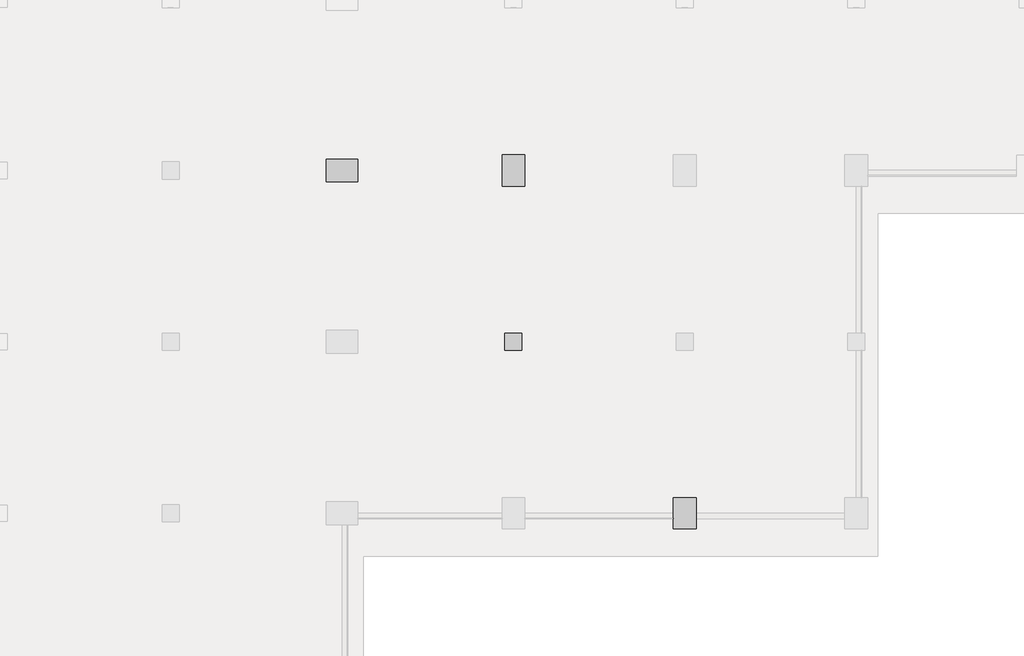
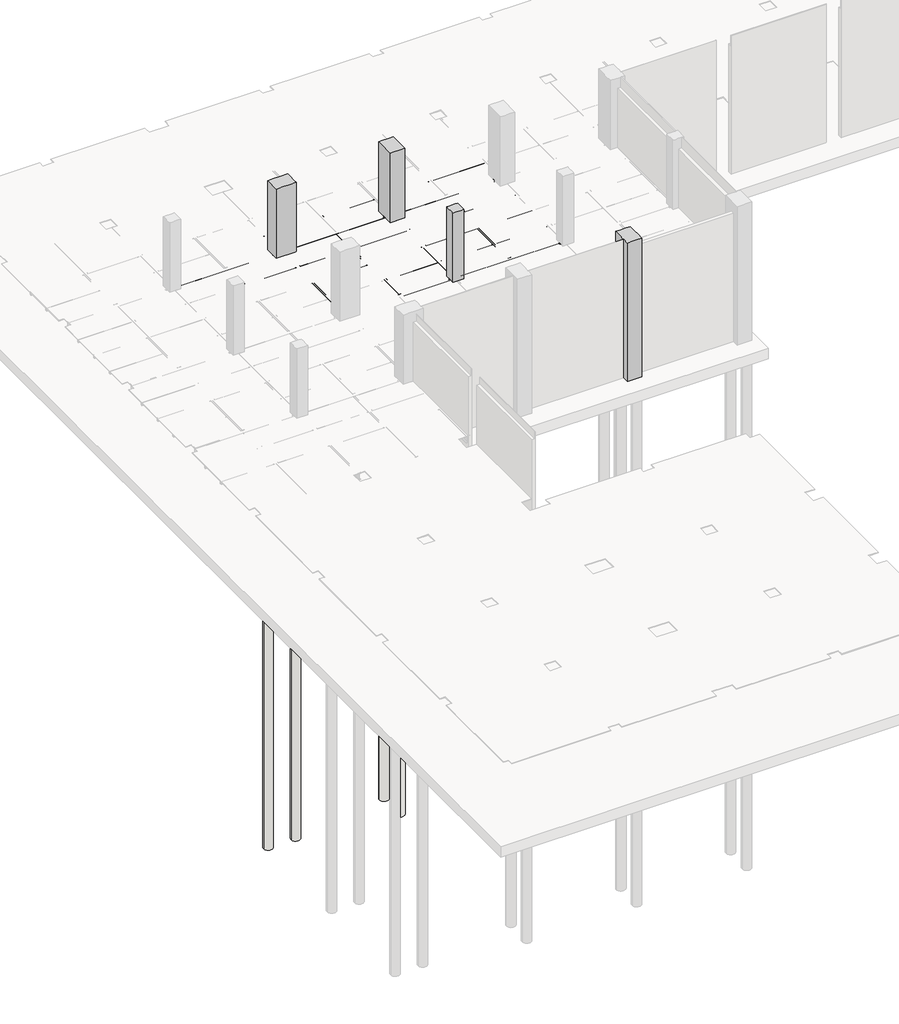
# Not in any storey, part 10 of 16: 28 beams, 6 slabs, 4 columns.
"""IFC4 building model written with IfcOpenShell, lengths in millimetres."""

from ifc_helpers import new_model, si_unit, point, frame, frame_2d, origin, place, context, project, spatial, polyline, circle_curve, trimmed, segment, composite_curve, outline, extrude, faceted_brep, element, save

model = new_model("IFC4")

# Units and contexts
model_context = context("Model", 3, world=origin())
ifc_project = project(units=[si_unit("LENGTHUNIT", "METRE", prefix="MILLI")], contexts=[model_context])

# Site, building
site = spatial("IfcSite", under=ifc_project)
building = spatial("IfcBuilding", under=site)

# Beams
placement = place(None, origin())
element("IfcBeam", 1, ObjectType="Steel Framing_H_KS : H_SB_AR_S02_H-400x200x8x13_BSG1", at=placement, inside=building, context=model_context, shape_type="SweptSolid", body=[
    extrude(outline(composite_curve([segment(polyline([(-17900.0, -4187.0381366), (-17900.0, -4200.0381366), (-18100.0, -4200.0381366), (-18100.0, -4187.0381366), (-18020.0, -4187.0381366)]), True, "CONTINUOUS"), segment(trimmed(circle_curve(frame_2d((-18020.0, -4171.0381366)), 16.0), [point((-18020.0, -4187.0381366))], [point((-18004.0, -4171.0381366))], True, "CARTESIAN"), True, "CONTINUOUS"), segment(polyline([(-18004.0, -4171.0381366), (-18004.0, -3829.0381366)]), True, "CONTINUOUS"), segment(trimmed(circle_curve(frame_2d((-18020.0, -3829.0381366)), 16.0), [point((-18004.0, -3829.0381366))], [point((-18020.0, -3813.0381366))], True, "CARTESIAN"), True, "CONTINUOUS"), segment(polyline([(-18020.0, -3813.0381366), (-18100.0, -3813.0381366), (-18100.0, -3800.0381366), (-17900.0, -3800.0381366), (-17900.0, -3813.0381366), (-17980.0, -3813.0381366)]), True, "CONTINUOUS"), segment(trimmed(circle_curve(frame_2d((-17980.0, -3829.0381366)), 16.0), [point((-17980.0, -3813.0381366))], [point((-17996.0, -3829.0381366))], True, "CARTESIAN"), True, "CONTINUOUS"), segment(polyline([(-17996.0, -3829.0381366), (-17996.0, -4171.0381366)]), True, "CONTINUOUS"), segment(trimmed(circle_curve(frame_2d((-17980.0, -4171.0381366)), 16.0), [point((-17996.0, -4171.0381366))], [point((-17980.0, -4187.0381366))], True, "CARTESIAN"), True, "CONTINUOUS"), segment(polyline([(-17980.0, -4187.0381366), (-17900.0, -4187.0381366)]), True, "CONTINUOUS")], self_intersect=False)), frame((30312.7, 0.0, 0.0), z_axis=(1.0, 0.0, 0.0), x_axis=(0.0, 1.0, 0.0)), (0.0, 0.0, 1.0), 5124.6),
])
element("IfcBeam", 2, ObjectType="Steel Framing_C_KS : H_SB_AR_S02_C-150x75x6.5x10_J1", at=placement, inside=building, context=model_context, shape_type="SweptSolid", body=[
    extrude(outline(composite_curve([segment(polyline([(-16477.2, -3800.0381366), (-16477.2, -3950.0381366), (-16552.2, -3950.0381366)]), True, "CONTINUOUS"), segment(trimmed(circle_curve(frame_2d((-16542.2, -3950.0381366)), 10.0), [point((-16552.2, -3950.0381366))], [point((-16542.2, -3940.0381366))], False, "CARTESIAN"), True, "CONTINUOUS"), segment(polyline([(-16542.2, -3940.0381366), (-16483.7, -3930.7726469), (-16483.7, -3819.3036264), (-16542.2, -3810.0381366)]), True, "CONTINUOUS"), segment(trimmed(circle_curve(frame_2d((-16542.2, -3800.0381366)), 10.0), [point((-16542.2, -3810.0381366))], [point((-16552.2, -3800.0381366))], False, "CARTESIAN"), True, "CONTINUOUS"), segment(polyline([(-16552.2, -3800.0381366), (-16477.2, -3800.0381366)]), True, "CONTINUOUS")], self_intersect=False)), frame((33112.7, 0.0, 0.0), z_axis=(1.0, 0.0, 0.0), x_axis=(0.0, 1.0, 0.0)), (0.0, 0.0, 1.0), 2774.6),
])
element("IfcBeam", 3, ObjectType="Steel Framing_H_KS : H_SB_AR_S02_H-400x200x8x13_BSG1", at=placement, inside=building, context=model_context, shape_type="SweptSolid", body=[
    extrude(outline(composite_curve([segment(polyline([(-17900.0, -4187.0381366), (-17900.0, -4200.0381366), (-18100.0, -4200.0381366), (-18100.0, -4187.0381366), (-18020.0, -4187.0381366)]), True, "CONTINUOUS"), segment(trimmed(circle_curve(frame_2d((-18020.0, -4171.0381366)), 16.0), [point((-18020.0, -4187.0381366))], [point((-18004.0, -4171.0381366))], True, "CARTESIAN"), True, "CONTINUOUS"), segment(polyline([(-18004.0, -4171.0381366), (-18004.0, -3829.0381366)]), True, "CONTINUOUS"), segment(trimmed(circle_curve(frame_2d((-18020.0, -3829.0381366)), 16.0), [point((-18004.0, -3829.0381366))], [point((-18020.0, -3813.0381366))], True, "CARTESIAN"), True, "CONTINUOUS"), segment(polyline([(-18020.0, -3813.0381366), (-18100.0, -3813.0381366), (-18100.0, -3800.0381366), (-17900.0, -3800.0381366), (-17900.0, -3813.0381366), (-17980.0, -3813.0381366)]), True, "CONTINUOUS"), segment(trimmed(circle_curve(frame_2d((-17980.0, -3829.0381366)), 16.0), [point((-17980.0, -3813.0381366))], [point((-17996.0, -3829.0381366))], True, "CARTESIAN"), True, "CONTINUOUS"), segment(polyline([(-17996.0, -3829.0381366), (-17996.0, -4171.0381366)]), True, "CONTINUOUS"), segment(trimmed(circle_curve(frame_2d((-17980.0, -4171.0381366)), 16.0), [point((-17996.0, -4171.0381366))], [point((-17980.0, -4187.0381366))], True, "CARTESIAN"), True, "CONTINUOUS"), segment(polyline([(-17980.0, -4187.0381366), (-17900.0, -4187.0381366)]), True, "CONTINUOUS")], self_intersect=False)), frame((36562.7, 0.0, 0.0), z_axis=(1.0, 0.0, 0.0), x_axis=(0.0, 1.0, 0.0)), (0.0, 0.0, 1.0), 5024.6),
])
element("IfcBeam", 4, ObjectType="Steel Framing_C_KS : H_SB_AR_S02_C-150x75x6.5x10_J1", at=placement, inside=building, context=model_context, shape_type="SweptSolid", body=[
    extrude(outline(composite_curve([segment(polyline([(-16477.2, -3800.0381366), (-16477.2, -3950.0381366), (-16552.2, -3950.0381366)]), True, "CONTINUOUS"), segment(trimmed(circle_curve(frame_2d((-16542.2, -3950.0381366)), 10.0), [point((-16552.2, -3950.0381366))], [point((-16542.2, -3940.0381366))], False, "CARTESIAN"), True, "CONTINUOUS"), segment(polyline([(-16542.2, -3940.0381366), (-16483.7, -3930.7726469), (-16483.7, -3819.3036264), (-16542.2, -3810.0381366)]), True, "CONTINUOUS"), segment(trimmed(circle_curve(frame_2d((-16542.2, -3800.0381366)), 10.0), [point((-16542.2, -3810.0381366))], [point((-16552.2, -3800.0381366))], False, "CARTESIAN"), True, "CONTINUOUS"), segment(polyline([(-16552.2, -3800.0381366), (-16477.2, -3800.0381366)]), True, "CONTINUOUS")], self_intersect=False)), frame((36112.7, 0.0, 0.0), z_axis=(1.0, 0.0, 0.0), x_axis=(0.0, 1.0, 0.0)), (0.0, 0.0, 1.0), 2774.6),
])
element("IfcBeam", 5, ObjectType="Steel Framing_C_KS : H_SB_AR_S02_C-150x75x6.5x10_J1", at=placement, inside=building, context=model_context, shape_type="SweptSolid", body=[
    extrude(outline(composite_curve([segment(polyline([(-16477.2, -3800.0381366), (-16477.2, -3950.0381366), (-16552.2, -3950.0381366)]), True, "CONTINUOUS"), segment(trimmed(circle_curve(frame_2d((-16542.2, -3950.0381366)), 10.0), [point((-16552.2, -3950.0381366))], [point((-16542.2, -3940.0381366))], False, "CARTESIAN"), True, "CONTINUOUS"), segment(polyline([(-16542.2, -3940.0381366), (-16483.7, -3930.7726469), (-16483.7, -3819.3036264), (-16542.2, -3810.0381366)]), True, "CONTINUOUS"), segment(trimmed(circle_curve(frame_2d((-16542.2, -3800.0381366)), 10.0), [point((-16542.2, -3810.0381366))], [point((-16552.2, -3800.0381366))], False, "CARTESIAN"), True, "CONTINUOUS"), segment(polyline([(-16552.2, -3800.0381366), (-16477.2, -3800.0381366)]), True, "CONTINUOUS")], self_intersect=False)), frame((39112.7, 0.0, 0.0), z_axis=(1.0, 0.0, 0.0), x_axis=(0.0, 1.0, 0.0)), (0.0, 0.0, 1.0), 2774.6),
])
element("IfcBeam", 6, ObjectType="Steel Framing_H_KS : H_SB_AR_S02_H-400x200x8x13_BSG1", at=placement, inside=building, context=model_context, shape_type="SweptSolid", body=[
    extrude(outline(composite_curve([segment(polyline([(-17900.0, -4187.0381366), (-17900.0, -4200.0381366), (-18100.0, -4200.0381366), (-18100.0, -4187.0381366), (-18020.0, -4187.0381366)]), True, "CONTINUOUS"), segment(trimmed(circle_curve(frame_2d((-18020.0, -4171.0381366)), 16.0), [point((-18020.0, -4187.0381366))], [point((-18004.0, -4171.0381366))], True, "CARTESIAN"), True, "CONTINUOUS"), segment(polyline([(-18004.0, -4171.0381366), (-18004.0, -3829.0381366)]), True, "CONTINUOUS"), segment(trimmed(circle_curve(frame_2d((-18020.0, -3829.0381366)), 16.0), [point((-18004.0, -3829.0381366))], [point((-18020.0, -3813.0381366))], True, "CARTESIAN"), True, "CONTINUOUS"), segment(polyline([(-18020.0, -3813.0381366), (-18100.0, -3813.0381366), (-18100.0, -3800.0381366), (-17900.0, -3800.0381366), (-17900.0, -3813.0381366), (-17980.0, -3813.0381366)]), True, "CONTINUOUS"), segment(trimmed(circle_curve(frame_2d((-17980.0, -3829.0381366)), 16.0), [point((-17980.0, -3813.0381366))], [point((-17996.0, -3829.0381366))], True, "CARTESIAN"), True, "CONTINUOUS"), segment(polyline([(-17996.0, -3829.0381366), (-17996.0, -4171.0381366)]), True, "CONTINUOUS"), segment(trimmed(circle_curve(frame_2d((-17980.0, -4171.0381366)), 16.0), [point((-17996.0, -4171.0381366))], [point((-17980.0, -4187.0381366))], True, "CARTESIAN"), True, "CONTINUOUS"), segment(polyline([(-17980.0, -4187.0381366), (-17900.0, -4187.0381366)]), True, "CONTINUOUS")], self_intersect=False)), frame((42412.7, 0.0, 0.0), z_axis=(1.0, 0.0, 0.0), x_axis=(0.0, 1.0, 0.0)), (0.0, 0.0, 1.0), 5174.6),
])
element("IfcBeam", 7, ObjectType="Steel Framing_C_KS : H_SB_AR_S02_C-150x75x6.5x10_J1", at=placement, inside=building, context=model_context, shape_type="SweptSolid", body=[
    extrude(outline(composite_curve([segment(polyline([(-16477.2, -3800.0381366), (-16477.2, -3950.0381366), (-16552.2, -3950.0381366)]), True, "CONTINUOUS"), segment(trimmed(circle_curve(frame_2d((-16542.2, -3950.0381366)), 10.0), [point((-16552.2, -3950.0381366))], [point((-16542.2, -3940.0381366))], False, "CARTESIAN"), True, "CONTINUOUS"), segment(polyline([(-16542.2, -3940.0381366), (-16483.7, -3930.7726469), (-16483.7, -3819.3036264), (-16542.2, -3810.0381366)]), True, "CONTINUOUS"), segment(trimmed(circle_curve(frame_2d((-16542.2, -3800.0381366)), 10.0), [point((-16542.2, -3810.0381366))], [point((-16552.2, -3800.0381366))], False, "CARTESIAN"), True, "CONTINUOUS"), segment(polyline([(-16552.2, -3800.0381366), (-16477.2, -3800.0381366)]), True, "CONTINUOUS")], self_intersect=False)), frame((42112.7, 0.0, 0.0), z_axis=(1.0, 0.0, 0.0), x_axis=(0.0, 1.0, 0.0)), (0.0, 0.0, 1.0), 2774.6),
])
element("IfcBeam", 8, ObjectType="Steel Framing_C_KS : H_SB_AR_S02_C-150x75x6.5x10_J1", at=placement, inside=building, context=model_context, shape_type="SweptSolid", body=[
    extrude(outline(composite_curve([segment(polyline([(-16477.2, -3800.0381366), (-16477.2, -3950.0381366), (-16552.2, -3950.0381366)]), True, "CONTINUOUS"), segment(trimmed(circle_curve(frame_2d((-16542.2, -3950.0381366)), 10.0), [point((-16552.2, -3950.0381366))], [point((-16542.2, -3940.0381366))], False, "CARTESIAN"), True, "CONTINUOUS"), segment(polyline([(-16542.2, -3940.0381366), (-16483.7, -3930.7726469), (-16483.7, -3819.3036264), (-16542.2, -3810.0381366)]), True, "CONTINUOUS"), segment(trimmed(circle_curve(frame_2d((-16542.2, -3800.0381366)), 10.0), [point((-16542.2, -3810.0381366))], [point((-16552.2, -3800.0381366))], False, "CARTESIAN"), True, "CONTINUOUS"), segment(polyline([(-16552.2, -3800.0381366), (-16477.2, -3800.0381366)]), True, "CONTINUOUS")], self_intersect=False)), frame((45112.7, 0.0, 0.0), z_axis=(1.0, 0.0, 0.0), x_axis=(0.0, 1.0, 0.0)), (0.0, 0.0, 1.0), 2774.6),
])
element("IfcBeam", 9, ObjectType="Steel Framing_H_KS : H_SB_AR_S02_H-400x200x8x13_BSG2", at=placement, inside=building, context=model_context, shape_type="SweptSolid", body=[
    extrude(outline(composite_curve([segment(polyline([(-4187.0381366, 35900.0), (-4200.0381366, 35900.0), (-4200.0381366, 36100.0), (-4187.0381366, 36100.0), (-4187.0381366, 36020.0)]), True, "CONTINUOUS"), segment(trimmed(circle_curve(frame_2d((-4171.0381366, 36020.0)), 16.0), [point((-4187.0381366, 36020.0))], [point((-4171.0381366, 36004.0))], True, "CARTESIAN"), True, "CONTINUOUS"), segment(polyline([(-4171.0381366, 36004.0), (-3829.0381366, 36004.0)]), True, "CONTINUOUS"), segment(trimmed(circle_curve(frame_2d((-3829.0381366, 36020.0)), 16.0), [point((-3829.0381366, 36004.0))], [point((-3813.0381366, 36020.0))], True, "CARTESIAN"), True, "CONTINUOUS"), segment(polyline([(-3813.0381366, 36020.0), (-3813.0381366, 36100.0), (-3800.0381366, 36100.0), (-3800.0381366, 35900.0), (-3813.0381366, 35900.0), (-3813.0381366, 35980.0)]), True, "CONTINUOUS"), segment(trimmed(circle_curve(frame_2d((-3829.0381366, 35980.0)), 16.0), [point((-3813.0381366, 35980.0))], [point((-3829.0381366, 35996.0))], True, "CARTESIAN"), True, "CONTINUOUS"), segment(polyline([(-3829.0381366, 35996.0), (-4171.0381366, 35996.0)]), True, "CONTINUOUS"), segment(trimmed(circle_curve(frame_2d((-4171.0381366, 35980.0)), 16.0), [point((-4171.0381366, 35996.0))], [point((-4187.0381366, 35980.0))], True, "CARTESIAN"), True, "CONTINUOUS"), segment(polyline([(-4187.0381366, 35980.0), (-4187.0381366, 35900.0)]), True, "CONTINUOUS")], self_intersect=False)), frame((0.0, -23587.3, 0.0), z_axis=(0.0, 1.0, 0.0), x_axis=(0.0, 0.0, 1.0)), (0.0, 0.0, 1.0), 5174.6),
])
element("IfcBeam", 10, ObjectType="Steel Framing_C_KS : H_SB_AR_S02_C-150x75x6.5x10_J1", at=placement, inside=building, context=model_context, shape_type="SweptSolid", body=[
    extrude(outline(composite_curve([segment(polyline([(-19477.2, -3800.0381366), (-19477.2, -3950.0381366), (-19552.2, -3950.0381366)]), True, "CONTINUOUS"), segment(trimmed(circle_curve(frame_2d((-19542.2, -3950.0381366)), 10.0), [point((-19552.2, -3950.0381366))], [point((-19542.2, -3940.0381366))], False, "CARTESIAN"), True, "CONTINUOUS"), segment(polyline([(-19542.2, -3940.0381366), (-19483.7, -3930.7726469), (-19483.7, -3819.3036264), (-19542.2, -3810.0381366)]), True, "CONTINUOUS"), segment(trimmed(circle_curve(frame_2d((-19542.2, -3800.0381366)), 10.0), [point((-19542.2, -3810.0381366))], [point((-19552.2, -3800.0381366))], False, "CARTESIAN"), True, "CONTINUOUS"), segment(polyline([(-19552.2, -3800.0381366), (-19477.2, -3800.0381366)]), True, "CONTINUOUS")], self_intersect=False)), frame((33112.7, 0.0, 0.0), z_axis=(1.0, 0.0, 0.0), x_axis=(0.0, 1.0, 0.0)), (0.0, 0.0, 1.0), 2774.6),
])
element("IfcBeam", 11, ObjectType="Steel Framing_H_KS : H_SB_AR_S02_H-400x200x8x13_BSG1", at=placement, inside=building, context=model_context, shape_type="SweptSolid", body=[
    extrude(outline(composite_curve([segment(polyline([(-23900.0, -4187.0381366), (-23900.0, -4200.0381366), (-24100.0, -4200.0381366), (-24100.0, -4187.0381366), (-24020.0, -4187.0381366)]), True, "CONTINUOUS"), segment(trimmed(circle_curve(frame_2d((-24020.0, -4171.0381366)), 16.0), [point((-24020.0, -4187.0381366))], [point((-24004.0, -4171.0381366))], True, "CARTESIAN"), True, "CONTINUOUS"), segment(polyline([(-24004.0, -4171.0381366), (-24004.0, -3829.0381366)]), True, "CONTINUOUS"), segment(trimmed(circle_curve(frame_2d((-24020.0, -3829.0381366)), 16.0), [point((-24004.0, -3829.0381366))], [point((-24020.0, -3813.0381366))], True, "CARTESIAN"), True, "CONTINUOUS"), segment(polyline([(-24020.0, -3813.0381366), (-24100.0, -3813.0381366), (-24100.0, -3800.0381366), (-23900.0, -3800.0381366), (-23900.0, -3813.0381366), (-23980.0, -3813.0381366)]), True, "CONTINUOUS"), segment(trimmed(circle_curve(frame_2d((-23980.0, -3829.0381366)), 16.0), [point((-23980.0, -3813.0381366))], [point((-23996.0, -3829.0381366))], True, "CARTESIAN"), True, "CONTINUOUS"), segment(polyline([(-23996.0, -3829.0381366), (-23996.0, -4171.0381366)]), True, "CONTINUOUS"), segment(trimmed(circle_curve(frame_2d((-23980.0, -4171.0381366)), 16.0), [point((-23996.0, -4171.0381366))], [point((-23980.0, -4187.0381366))], True, "CARTESIAN"), True, "CONTINUOUS"), segment(polyline([(-23980.0, -4187.0381366), (-23900.0, -4187.0381366)]), True, "CONTINUOUS")], self_intersect=False)), frame((36562.7, 0.0, 0.0), z_axis=(1.0, 0.0, 0.0), x_axis=(0.0, 1.0, 0.0)), (0.0, 0.0, 1.0), 5124.6),
])
element("IfcBeam", 12, ObjectType="Steel Framing_H_KS : H_SB_AR_S02_H-400x200x8x13_BSG2", at=placement, inside=building, context=model_context, shape_type="SweptSolid", body=[
    extrude(outline(composite_curve([segment(polyline([(-4187.0381366, 41900.0), (-4200.0381366, 41900.0), (-4200.0381366, 42100.0), (-4187.0381366, 42100.0), (-4187.0381366, 42020.0)]), True, "CONTINUOUS"), segment(trimmed(circle_curve(frame_2d((-4171.0381366, 42020.0)), 16.0), [point((-4187.0381366, 42020.0))], [point((-4171.0381366, 42004.0))], True, "CARTESIAN"), True, "CONTINUOUS"), segment(polyline([(-4171.0381366, 42004.0), (-3829.0381366, 42004.0)]), True, "CONTINUOUS"), segment(trimmed(circle_curve(frame_2d((-3829.0381366, 42020.0)), 16.0), [point((-3829.0381366, 42004.0))], [point((-3813.0381366, 42020.0))], True, "CARTESIAN"), True, "CONTINUOUS"), segment(polyline([(-3813.0381366, 42020.0), (-3813.0381366, 42100.0), (-3800.0381366, 42100.0), (-3800.0381366, 41900.0), (-3813.0381366, 41900.0), (-3813.0381366, 41980.0)]), True, "CONTINUOUS"), segment(trimmed(circle_curve(frame_2d((-3829.0381366, 41980.0)), 16.0), [point((-3813.0381366, 41980.0))], [point((-3829.0381366, 41996.0))], True, "CARTESIAN"), True, "CONTINUOUS"), segment(polyline([(-3829.0381366, 41996.0), (-4171.0381366, 41996.0)]), True, "CONTINUOUS"), segment(trimmed(circle_curve(frame_2d((-4171.0381366, 41980.0)), 16.0), [point((-4171.0381366, 41996.0))], [point((-4187.0381366, 41980.0))], True, "CARTESIAN"), True, "CONTINUOUS"), segment(polyline([(-4187.0381366, 41980.0), (-4187.0381366, 41900.0)]), True, "CONTINUOUS")], self_intersect=False)), frame((0.0, -23687.3, 0.0), z_axis=(0.0, 1.0, 0.0), x_axis=(0.0, 0.0, 1.0)), (0.0, 0.0, 1.0), 5124.6),
])
element("IfcBeam", 13, ObjectType="Steel Framing_H_KS : H_SB_AR_S02_H-400x200x8x13_BSB1", at=placement, inside=building, context=model_context, shape_type="SweptSolid", body=[
    extrude(outline(composite_curve([segment(polyline([(-4187.0381366, 38900.0), (-4200.0381366, 38900.0), (-4200.0381366, 39100.0), (-4187.0381366, 39100.0), (-4187.0381366, 39020.0)]), True, "CONTINUOUS"), segment(trimmed(circle_curve(frame_2d((-4171.0381366, 39020.0)), 16.0), [point((-4187.0381366, 39020.0))], [point((-4171.0381366, 39004.0))], True, "CARTESIAN"), True, "CONTINUOUS"), segment(polyline([(-4171.0381366, 39004.0), (-3829.0381366, 39004.0)]), True, "CONTINUOUS"), segment(trimmed(circle_curve(frame_2d((-3829.0381366, 39020.0)), 16.0), [point((-3829.0381366, 39004.0))], [point((-3813.0381366, 39020.0))], True, "CARTESIAN"), True, "CONTINUOUS"), segment(polyline([(-3813.0381366, 39020.0), (-3813.0381366, 39100.0), (-3800.0381366, 39100.0), (-3800.0381366, 38900.0), (-3813.0381366, 38900.0), (-3813.0381366, 38980.0)]), True, "CONTINUOUS"), segment(trimmed(circle_curve(frame_2d((-3829.0381366, 38980.0)), 16.0), [point((-3813.0381366, 38980.0))], [point((-3829.0381366, 38996.0))], True, "CARTESIAN"), True, "CONTINUOUS"), segment(polyline([(-3829.0381366, 38996.0), (-4171.0381366, 38996.0)]), True, "CONTINUOUS"), segment(trimmed(circle_curve(frame_2d((-4171.0381366, 38980.0)), 16.0), [point((-4171.0381366, 38996.0))], [point((-4187.0381366, 38980.0))], True, "CARTESIAN"), True, "CONTINUOUS"), segment(polyline([(-4187.0381366, 38980.0), (-4187.0381366, 38900.0)]), True, "CONTINUOUS")], self_intersect=False)), frame((0.0, -23887.3, 0.0), z_axis=(0.0, 1.0, 0.0), x_axis=(0.0, 0.0, 1.0)), (0.0, 0.0, 1.0), 5774.6),
])
element("IfcBeam", 14, ObjectType="Steel Framing_C_KS : H_SB_AR_S02_C-150x75x6.5x10_J1", at=placement, inside=building, context=model_context, shape_type="SweptSolid", body=[
    extrude(outline(composite_curve([segment(polyline([(-20977.2, -3800.0381366), (-20977.2, -3950.0381366), (-21052.2, -3950.0381366)]), True, "CONTINUOUS"), segment(trimmed(circle_curve(frame_2d((-21042.2, -3950.0381366)), 10.0), [point((-21052.2, -3950.0381366))], [point((-21042.2, -3940.0381366))], False, "CARTESIAN"), True, "CONTINUOUS"), segment(polyline([(-21042.2, -3940.0381366), (-20983.7, -3930.7726469), (-20983.7, -3819.3036264), (-21042.2, -3810.0381366)]), True, "CONTINUOUS"), segment(trimmed(circle_curve(frame_2d((-21042.2, -3800.0381366)), 10.0), [point((-21042.2, -3810.0381366))], [point((-21052.2, -3800.0381366))], False, "CARTESIAN"), True, "CONTINUOUS"), segment(polyline([(-21052.2, -3800.0381366), (-20977.2, -3800.0381366)]), True, "CONTINUOUS")], self_intersect=False)), frame((36112.7, 0.0, 0.0), z_axis=(1.0, 0.0, 0.0), x_axis=(0.0, 1.0, 0.0)), (0.0, 0.0, 1.0), 2774.6),
])
element("IfcBeam", 15, ObjectType="Steel Framing_C_KS : H_SB_AR_S02_C-150x75x6.5x10_J1", at=placement, inside=building, context=model_context, shape_type="SweptSolid", body=[
    extrude(outline(composite_curve([segment(polyline([(-19477.2, -3800.0381366), (-19477.2, -3950.0381366), (-19552.2, -3950.0381366)]), True, "CONTINUOUS"), segment(trimmed(circle_curve(frame_2d((-19542.2, -3950.0381366)), 10.0), [point((-19552.2, -3950.0381366))], [point((-19542.2, -3940.0381366))], False, "CARTESIAN"), True, "CONTINUOUS"), segment(polyline([(-19542.2, -3940.0381366), (-19483.7, -3930.7726469), (-19483.7, -3819.3036264), (-19542.2, -3810.0381366)]), True, "CONTINUOUS"), segment(trimmed(circle_curve(frame_2d((-19542.2, -3800.0381366)), 10.0), [point((-19542.2, -3810.0381366))], [point((-19552.2, -3800.0381366))], False, "CARTESIAN"), True, "CONTINUOUS"), segment(polyline([(-19552.2, -3800.0381366), (-19477.2, -3800.0381366)]), True, "CONTINUOUS")], self_intersect=False)), frame((36112.7, 0.0, 0.0), z_axis=(1.0, 0.0, 0.0), x_axis=(0.0, 1.0, 0.0)), (0.0, 0.0, 1.0), 2774.6),
])
element("IfcBeam", 16, ObjectType="Steel Framing_C_KS : H_SB_AR_S02_C-150x75x6.5x10_J1", at=placement, inside=building, context=model_context, shape_type="SweptSolid", body=[
    extrude(outline(composite_curve([segment(polyline([(-20977.2, -3800.0381366), (-20977.2, -3950.0381366), (-21052.2, -3950.0381366)]), True, "CONTINUOUS"), segment(trimmed(circle_curve(frame_2d((-21042.2, -3950.0381366)), 10.0), [point((-21052.2, -3950.0381366))], [point((-21042.2, -3940.0381366))], False, "CARTESIAN"), True, "CONTINUOUS"), segment(polyline([(-21042.2, -3940.0381366), (-20983.7, -3930.7726469), (-20983.7, -3819.3036264), (-21042.2, -3810.0381366)]), True, "CONTINUOUS"), segment(trimmed(circle_curve(frame_2d((-21042.2, -3800.0381366)), 10.0), [point((-21042.2, -3810.0381366))], [point((-21052.2, -3800.0381366))], False, "CARTESIAN"), True, "CONTINUOUS"), segment(polyline([(-21052.2, -3800.0381366), (-20977.2, -3800.0381366)]), True, "CONTINUOUS")], self_intersect=False)), frame((39112.7, 0.0, 0.0), z_axis=(1.0, 0.0, 0.0), x_axis=(0.0, 1.0, 0.0)), (0.0, 0.0, 1.0), 2774.6),
])
element("IfcBeam", 17, ObjectType="Steel Framing_C_KS : H_SB_AR_S02_C-150x75x6.5x10_J1", at=placement, inside=building, context=model_context, shape_type="SweptSolid", body=[
    extrude(outline(composite_curve([segment(polyline([(-22477.2, -3800.0381366), (-22477.2, -3950.0381366), (-22552.2, -3950.0381366)]), True, "CONTINUOUS"), segment(trimmed(circle_curve(frame_2d((-22542.2, -3950.0381366)), 10.0), [point((-22552.2, -3950.0381366))], [point((-22542.2, -3940.0381366))], False, "CARTESIAN"), True, "CONTINUOUS"), segment(polyline([(-22542.2, -3940.0381366), (-22483.7, -3930.7726469), (-22483.7, -3819.3036264), (-22542.2, -3810.0381366)]), True, "CONTINUOUS"), segment(trimmed(circle_curve(frame_2d((-22542.2, -3800.0381366)), 10.0), [point((-22542.2, -3810.0381366))], [point((-22552.2, -3800.0381366))], False, "CARTESIAN"), True, "CONTINUOUS"), segment(polyline([(-22552.2, -3800.0381366), (-22477.2, -3800.0381366)]), True, "CONTINUOUS")], self_intersect=False)), frame((39112.7, 0.0, 0.0), z_axis=(1.0, 0.0, 0.0), x_axis=(0.0, 1.0, 0.0)), (0.0, 0.0, 1.0), 2774.6),
])
element("IfcBeam", 18, ObjectType="Steel Framing_C_KS : H_SB_AR_S02_C-150x75x6.5x10_J1", at=placement, inside=building, context=model_context, shape_type="SweptSolid", body=[
    extrude(outline(composite_curve([segment(polyline([(-19477.2, -3800.0381366), (-19477.2, -3950.0381366), (-19552.2, -3950.0381366)]), True, "CONTINUOUS"), segment(trimmed(circle_curve(frame_2d((-19542.2, -3950.0381366)), 10.0), [point((-19552.2, -3950.0381366))], [point((-19542.2, -3940.0381366))], False, "CARTESIAN"), True, "CONTINUOUS"), segment(polyline([(-19542.2, -3940.0381366), (-19483.7, -3930.7726469), (-19483.7, -3819.3036264), (-19542.2, -3810.0381366)]), True, "CONTINUOUS"), segment(trimmed(circle_curve(frame_2d((-19542.2, -3800.0381366)), 10.0), [point((-19542.2, -3810.0381366))], [point((-19552.2, -3800.0381366))], False, "CARTESIAN"), True, "CONTINUOUS"), segment(polyline([(-19552.2, -3800.0381366), (-19477.2, -3800.0381366)]), True, "CONTINUOUS")], self_intersect=False)), frame((39112.7, 0.0, 0.0), z_axis=(1.0, 0.0, 0.0), x_axis=(0.0, 1.0, 0.0)), (0.0, 0.0, 1.0), 2774.6),
])
element("IfcBeam", 19, ObjectType="Steel Framing_H_KS : H_SB_AR_S02_H-400x200x8x13_BSG1", at=placement, inside=building, context=model_context, shape_type="SweptSolid", body=[
    extrude(outline(composite_curve([segment(polyline([(-23900.0, -4187.0381366), (-23900.0, -4200.0381366), (-24100.0, -4200.0381366), (-24100.0, -4187.0381366), (-24020.0, -4187.0381366)]), True, "CONTINUOUS"), segment(trimmed(circle_curve(frame_2d((-24020.0, -4171.0381366)), 16.0), [point((-24020.0, -4187.0381366))], [point((-24004.0, -4171.0381366))], True, "CARTESIAN"), True, "CONTINUOUS"), segment(polyline([(-24004.0, -4171.0381366), (-24004.0, -3829.0381366)]), True, "CONTINUOUS"), segment(trimmed(circle_curve(frame_2d((-24020.0, -3829.0381366)), 16.0), [point((-24004.0, -3829.0381366))], [point((-24020.0, -3813.0381366))], True, "CARTESIAN"), True, "CONTINUOUS"), segment(polyline([(-24020.0, -3813.0381366), (-24100.0, -3813.0381366), (-24100.0, -3800.0381366), (-23900.0, -3800.0381366), (-23900.0, -3813.0381366), (-23980.0, -3813.0381366)]), True, "CONTINUOUS"), segment(trimmed(circle_curve(frame_2d((-23980.0, -3829.0381366)), 16.0), [point((-23980.0, -3813.0381366))], [point((-23996.0, -3829.0381366))], True, "CARTESIAN"), True, "CONTINUOUS"), segment(polyline([(-23996.0, -3829.0381366), (-23996.0, -4171.0381366)]), True, "CONTINUOUS"), segment(trimmed(circle_curve(frame_2d((-23980.0, -4171.0381366)), 16.0), [point((-23996.0, -4171.0381366))], [point((-23980.0, -4187.0381366))], True, "CARTESIAN"), True, "CONTINUOUS"), segment(polyline([(-23980.0, -4187.0381366), (-23900.0, -4187.0381366)]), True, "CONTINUOUS")], self_intersect=False)), frame((42312.7, 0.0, 0.0), z_axis=(1.0, 0.0, 0.0), x_axis=(0.0, 1.0, 0.0)), (0.0, 0.0, 1.0), 5374.6),
])
element("IfcBeam", 20, ObjectType="Steel Framing_H_KS : H_SB_AR_S02_H-400x200x8x13_BSB1", at=placement, inside=building, context=model_context, shape_type="SweptSolid", body=[
    extrude(outline(composite_curve([segment(polyline([(-4187.0381366, 44900.0), (-4200.0381366, 44900.0), (-4200.0381366, 45100.0), (-4187.0381366, 45100.0), (-4187.0381366, 45020.0)]), True, "CONTINUOUS"), segment(trimmed(circle_curve(frame_2d((-4171.0381366, 45020.0)), 16.0), [point((-4187.0381366, 45020.0))], [point((-4171.0381366, 45004.0))], True, "CARTESIAN"), True, "CONTINUOUS"), segment(polyline([(-4171.0381366, 45004.0), (-3829.0381366, 45004.0)]), True, "CONTINUOUS"), segment(trimmed(circle_curve(frame_2d((-3829.0381366, 45020.0)), 16.0), [point((-3829.0381366, 45004.0))], [point((-3813.0381366, 45020.0))], True, "CARTESIAN"), True, "CONTINUOUS"), segment(polyline([(-3813.0381366, 45020.0), (-3813.0381366, 45100.0), (-3800.0381366, 45100.0), (-3800.0381366, 44900.0), (-3813.0381366, 44900.0), (-3813.0381366, 44980.0)]), True, "CONTINUOUS"), segment(trimmed(circle_curve(frame_2d((-3829.0381366, 44980.0)), 16.0), [point((-3813.0381366, 44980.0))], [point((-3829.0381366, 44996.0))], True, "CARTESIAN"), True, "CONTINUOUS"), segment(polyline([(-3829.0381366, 44996.0), (-4171.0381366, 44996.0)]), True, "CONTINUOUS"), segment(trimmed(circle_curve(frame_2d((-4171.0381366, 44980.0)), 16.0), [point((-4171.0381366, 44996.0))], [point((-4187.0381366, 44980.0))], True, "CARTESIAN"), True, "CONTINUOUS"), segment(polyline([(-4187.0381366, 44980.0), (-4187.0381366, 44900.0)]), True, "CONTINUOUS")], self_intersect=False)), frame((0.0, -23887.3, 0.0), z_axis=(0.0, 1.0, 0.0), x_axis=(0.0, 0.0, 1.0)), (0.0, 0.0, 1.0), 5774.6),
])
element("IfcBeam", 21, ObjectType="Steel Framing_C_KS : H_SB_AR_S02_C-150x75x6.5x10_J1", at=placement, inside=building, context=model_context, shape_type="SweptSolid", body=[
    extrude(outline(composite_curve([segment(polyline([(-20977.2, -3800.0381366), (-20977.2, -3950.0381366), (-21052.2, -3950.0381366)]), True, "CONTINUOUS"), segment(trimmed(circle_curve(frame_2d((-21042.2, -3950.0381366)), 10.0), [point((-21052.2, -3950.0381366))], [point((-21042.2, -3940.0381366))], False, "CARTESIAN"), True, "CONTINUOUS"), segment(polyline([(-21042.2, -3940.0381366), (-20983.7, -3930.7726469), (-20983.7, -3819.3036264), (-21042.2, -3810.0381366)]), True, "CONTINUOUS"), segment(trimmed(circle_curve(frame_2d((-21042.2, -3800.0381366)), 10.0), [point((-21042.2, -3810.0381366))], [point((-21052.2, -3800.0381366))], False, "CARTESIAN"), True, "CONTINUOUS"), segment(polyline([(-21052.2, -3800.0381366), (-20977.2, -3800.0381366)]), True, "CONTINUOUS")], self_intersect=False)), frame((42112.7, 0.0, 0.0), z_axis=(1.0, 0.0, 0.0), x_axis=(0.0, 1.0, 0.0)), (0.0, 0.0, 1.0), 2774.6),
])
element("IfcBeam", 22, ObjectType="Steel Framing_C_KS : H_SB_AR_S02_C-150x75x6.5x10_J1", at=placement, inside=building, context=model_context, shape_type="SweptSolid", body=[
    extrude(outline(composite_curve([segment(polyline([(-22477.2, -3800.0381366), (-22477.2, -3950.0381366), (-22552.2, -3950.0381366)]), True, "CONTINUOUS"), segment(trimmed(circle_curve(frame_2d((-22542.2, -3950.0381366)), 10.0), [point((-22552.2, -3950.0381366))], [point((-22542.2, -3940.0381366))], False, "CARTESIAN"), True, "CONTINUOUS"), segment(polyline([(-22542.2, -3940.0381366), (-22483.7, -3930.7726469), (-22483.7, -3819.3036264), (-22542.2, -3810.0381366)]), True, "CONTINUOUS"), segment(trimmed(circle_curve(frame_2d((-22542.2, -3800.0381366)), 10.0), [point((-22542.2, -3810.0381366))], [point((-22552.2, -3800.0381366))], False, "CARTESIAN"), True, "CONTINUOUS"), segment(polyline([(-22552.2, -3800.0381366), (-22477.2, -3800.0381366)]), True, "CONTINUOUS")], self_intersect=False)), frame((42112.7, 0.0, 0.0), z_axis=(1.0, 0.0, 0.0), x_axis=(0.0, 1.0, 0.0)), (0.0, 0.0, 1.0), 2774.6),
])
element("IfcBeam", 23, ObjectType="Steel Framing_C_KS : H_SB_AR_S02_C-150x75x6.5x10_J1", at=placement, inside=building, context=model_context, shape_type="SweptSolid", body=[
    extrude(outline(composite_curve([segment(polyline([(-19477.2, -3800.0381366), (-19477.2, -3950.0381366), (-19552.2, -3950.0381366)]), True, "CONTINUOUS"), segment(trimmed(circle_curve(frame_2d((-19542.2, -3950.0381366)), 10.0), [point((-19552.2, -3950.0381366))], [point((-19542.2, -3940.0381366))], False, "CARTESIAN"), True, "CONTINUOUS"), segment(polyline([(-19542.2, -3940.0381366), (-19483.7, -3930.7726469), (-19483.7, -3819.3036264), (-19542.2, -3810.0381366)]), True, "CONTINUOUS"), segment(trimmed(circle_curve(frame_2d((-19542.2, -3800.0381366)), 10.0), [point((-19542.2, -3810.0381366))], [point((-19552.2, -3800.0381366))], False, "CARTESIAN"), True, "CONTINUOUS"), segment(polyline([(-19552.2, -3800.0381366), (-19477.2, -3800.0381366)]), True, "CONTINUOUS")], self_intersect=False)), frame((42112.7, 0.0, 0.0), z_axis=(1.0, 0.0, 0.0), x_axis=(0.0, 1.0, 0.0)), (0.0, 0.0, 1.0), 2774.6),
])
element("IfcBeam", 24, ObjectType="Steel Framing_C_KS : H_SB_AR_S02_C-150x75x6.5x10_J1", at=placement, inside=building, context=model_context, shape_type="SweptSolid", body=[
    extrude(outline(composite_curve([segment(polyline([(-20977.2, -3800.0381366), (-20977.2, -3950.0381366), (-21052.2, -3950.0381366)]), True, "CONTINUOUS"), segment(trimmed(circle_curve(frame_2d((-21042.2, -3950.0381366)), 10.0), [point((-21052.2, -3950.0381366))], [point((-21042.2, -3940.0381366))], False, "CARTESIAN"), True, "CONTINUOUS"), segment(polyline([(-21042.2, -3940.0381366), (-20983.7, -3930.7726469), (-20983.7, -3819.3036264), (-21042.2, -3810.0381366)]), True, "CONTINUOUS"), segment(trimmed(circle_curve(frame_2d((-21042.2, -3800.0381366)), 10.0), [point((-21042.2, -3810.0381366))], [point((-21052.2, -3800.0381366))], False, "CARTESIAN"), True, "CONTINUOUS"), segment(polyline([(-21052.2, -3800.0381366), (-20977.2, -3800.0381366)]), True, "CONTINUOUS")], self_intersect=False)), frame((45112.7, 0.0, 0.0), z_axis=(1.0, 0.0, 0.0), x_axis=(0.0, 1.0, 0.0)), (0.0, 0.0, 1.0), 2774.6),
])
element("IfcBeam", 25, ObjectType="Steel Framing_C_KS : H_SB_AR_S02_C-150x75x6.5x10_J1", at=placement, inside=building, context=model_context, shape_type="SweptSolid", body=[
    extrude(outline(composite_curve([segment(polyline([(-22477.2, -3800.0381366), (-22477.2, -3950.0381366), (-22552.2, -3950.0381366)]), True, "CONTINUOUS"), segment(trimmed(circle_curve(frame_2d((-22542.2, -3950.0381366)), 10.0), [point((-22552.2, -3950.0381366))], [point((-22542.2, -3940.0381366))], False, "CARTESIAN"), True, "CONTINUOUS"), segment(polyline([(-22542.2, -3940.0381366), (-22483.7, -3930.7726469), (-22483.7, -3819.3036264), (-22542.2, -3810.0381366)]), True, "CONTINUOUS"), segment(trimmed(circle_curve(frame_2d((-22542.2, -3800.0381366)), 10.0), [point((-22542.2, -3810.0381366))], [point((-22552.2, -3800.0381366))], False, "CARTESIAN"), True, "CONTINUOUS"), segment(polyline([(-22552.2, -3800.0381366), (-22477.2, -3800.0381366)]), True, "CONTINUOUS")], self_intersect=False)), frame((45112.7, 0.0, 0.0), z_axis=(1.0, 0.0, 0.0), x_axis=(0.0, 1.0, 0.0)), (0.0, 0.0, 1.0), 2774.6),
])
element("IfcBeam", 26, ObjectType="Steel Framing_C_KS : H_SB_AR_S02_C-150x75x6.5x10_J1", at=placement, inside=building, context=model_context, shape_type="SweptSolid", body=[
    extrude(outline(composite_curve([segment(polyline([(-19477.2, -3800.0381366), (-19477.2, -3950.0381366), (-19552.2, -3950.0381366)]), True, "CONTINUOUS"), segment(trimmed(circle_curve(frame_2d((-19542.2, -3950.0381366)), 10.0), [point((-19552.2, -3950.0381366))], [point((-19542.2, -3940.0381366))], False, "CARTESIAN"), True, "CONTINUOUS"), segment(polyline([(-19542.2, -3940.0381366), (-19483.7, -3930.7726469), (-19483.7, -3819.3036264), (-19542.2, -3810.0381366)]), True, "CONTINUOUS"), segment(trimmed(circle_curve(frame_2d((-19542.2, -3800.0381366)), 10.0), [point((-19542.2, -3810.0381366))], [point((-19552.2, -3800.0381366))], False, "CARTESIAN"), True, "CONTINUOUS"), segment(polyline([(-19552.2, -3800.0381366), (-19477.2, -3800.0381366)]), True, "CONTINUOUS")], self_intersect=False)), frame((45112.7, 0.0, 0.0), z_axis=(1.0, 0.0, 0.0), x_axis=(0.0, 1.0, 0.0)), (0.0, 0.0, 1.0), 2774.6),
])
element("IfcBeam", 27, ObjectType="Steel Framing_H_KS : H_SB_AR_S02_H-400x200x8x13_BSG1", at=placement, inside=building, context=model_context, shape_type="SweptSolid", body=[
    extrude(outline(composite_curve([segment(polyline([(-29900.0, -4187.0381366), (-29900.0, -4200.0381366), (-30100.0, -4200.0381366), (-30100.0, -4187.0381366), (-30020.0, -4187.0381366)]), True, "CONTINUOUS"), segment(trimmed(circle_curve(frame_2d((-30020.0, -4171.0381366)), 16.0), [point((-30020.0, -4187.0381366))], [point((-30004.0, -4171.0381366))], True, "CARTESIAN"), True, "CONTINUOUS"), segment(polyline([(-30004.0, -4171.0381366), (-30004.0, -3829.0381366)]), True, "CONTINUOUS"), segment(trimmed(circle_curve(frame_2d((-30020.0, -3829.0381366)), 16.0), [point((-30004.0, -3829.0381366))], [point((-30020.0, -3813.0381366))], True, "CARTESIAN"), True, "CONTINUOUS"), segment(polyline([(-30020.0, -3813.0381366), (-30100.0, -3813.0381366), (-30100.0, -3800.0381366), (-29900.0, -3800.0381366), (-29900.0, -3813.0381366), (-29980.0, -3813.0381366)]), True, "CONTINUOUS"), segment(trimmed(circle_curve(frame_2d((-29980.0, -3829.0381366)), 16.0), [point((-29980.0, -3813.0381366))], [point((-29996.0, -3829.0381366))], True, "CARTESIAN"), True, "CONTINUOUS"), segment(polyline([(-29996.0, -3829.0381366), (-29996.0, -4171.0381366)]), True, "CONTINUOUS"), segment(trimmed(circle_curve(frame_2d((-29980.0, -4171.0381366)), 16.0), [point((-29996.0, -4171.0381366))], [point((-29980.0, -4187.0381366))], True, "CARTESIAN"), True, "CONTINUOUS"), segment(polyline([(-29980.0, -4187.0381366), (-29900.0, -4187.0381366)]), True, "CONTINUOUS")], self_intersect=False)), frame((48412.7, 0.0, 0.0), z_axis=(1.0, 0.0, 0.0), x_axis=(0.0, 1.0, 0.0)), (0.0, 0.0, 1.0), 5174.6),
])
element("IfcBeam", 28, ObjectType="Steel Framing_C_KS : H_SB_AR_S02_C-150x75x6.5x10_J1", at=placement, inside=building, context=model_context, shape_type="SweptSolid", body=[
    extrude(outline(composite_curve([segment(polyline([(-28477.2, -3800.0381366), (-28477.2, -3950.0381366), (-28552.2, -3950.0381366)]), True, "CONTINUOUS"), segment(trimmed(circle_curve(frame_2d((-28542.2, -3950.0381366)), 10.0), [point((-28552.2, -3950.0381366))], [point((-28542.2, -3940.0381366))], False, "CARTESIAN"), True, "CONTINUOUS"), segment(polyline([(-28542.2, -3940.0381366), (-28483.7, -3930.7726469), (-28483.7, -3819.3036264), (-28542.2, -3810.0381366)]), True, "CONTINUOUS"), segment(trimmed(circle_curve(frame_2d((-28542.2, -3800.0381366)), 10.0), [point((-28542.2, -3810.0381366))], [point((-28552.2, -3800.0381366))], False, "CARTESIAN"), True, "CONTINUOUS"), segment(polyline([(-28552.2, -3800.0381366), (-28477.2, -3800.0381366)]), True, "CONTINUOUS")], self_intersect=False)), frame((48112.7, 0.0, 0.0), z_axis=(1.0, 0.0, 0.0), x_axis=(0.0, 1.0, 0.0)), (0.0, 0.0, 1.0), 2774.6),
])

# Columns
element("IfcColumn", 29, ObjectType="RC_Column_Rectangular : H_SC_AR_S15_UG PED_Bit_800x1100_PD1", at=placement, inside=building, context=model_context, shape_type="Brep", body=[
    faceted_brep([(35450.0, -17600.0, -7800.0381366), (36550.0, -17600.0, -7800.0381366), (36550.0, -18400.0, -7800.0381366), (35450.0, -18400.0, -7800.0381366), (35450.0, -17600.0, 199.9618634), (35825.0, -17600.0, 199.9618634), (36175.0, -17600.0, 199.9618634), (36550.0, -17600.0, 199.9618634), (36550.0, -17600.0, -0.0381366), (36550.0, -17600.0, -3800.0381366), (36550.0, -17600.0, -3832.0381366), (35450.0, -17600.0, -3832.0381366), (35450.0, -17600.0, -3800.0381366), (35450.0, -17600.0, -0.0381366), (36550.0, -17825.0, 199.9618634), (36550.0, -18175.0, 199.9618634), (36550.0, -18400.0, 199.9618634), (36550.0, -18400.0, -0.0381366), (36550.0, -18400.0, -3800.0381366), (36550.0, -18400.0, -3832.0381366), (36175.0, -18400.0, 199.9618634), (35825.0, -18400.0, 199.9618634), (35450.0, -18400.0, 199.9618634), (35450.0, -18400.0, -0.0381366), (35450.0, -18400.0, -3800.0381366), (35450.0, -18400.0, -3832.0381366), (35450.0, -18175.0, 199.9618634), (35450.0, -17825.0, 199.9618634)], [[[0, 1, 2, 3]], [[4, 5, 6, 7, 8, 9, 10, 1, 0, 11, 12, 13]], [[7, 14, 15, 16, 17, 18, 19, 2, 1, 10, 9, 8]], [[16, 20, 21, 22, 23, 24, 25, 3, 2, 19, 18, 17]], [[22, 26, 27, 4, 13, 12, 11, 0, 3, 25, 24, 23]], [[4, 27, 26, 22, 21, 20, 16, 15, 14, 7, 6, 5]]]),
])
element("IfcColumn", 30, ObjectType="RC_Column_Rectangular : H_SC_AR_S15_UG PED_Bit_800x1100_PD1", at=placement, inside=building, context=model_context, shape_type="Brep", body=[
    faceted_brep([(42400.0, -17450.0, -7800.0381366), (42400.0, -18550.0, -7800.0381366), (41600.0, -18550.0, -7800.0381366), (41600.0, -17450.0, -7800.0381366), (42400.0, -17450.0, 199.9618634), (42400.0, -17825.0, 199.9618634), (42400.0, -18175.0, 199.9618634), (42400.0, -18550.0, 199.9618634), (42400.0, -18550.0, -0.0381366), (42400.0, -18550.0, -3800.0381366), (42400.0, -18550.0, -3832.0381366), (42400.0, -17450.0, -3832.0381366), (42400.0, -17450.0, -3800.0381366), (42400.0, -17450.0, -0.0381366), (42175.0, -18550.0, 199.9618634), (41825.0, -18550.0, 199.9618634), (41600.0, -18550.0, 199.9618634), (41600.0, -18550.0, -0.0381366), (41600.0, -18550.0, -3800.0381366), (41600.0, -18550.0, -3832.0381366), (41600.0, -18175.0, 199.9618634), (41600.0, -17825.0, 199.9618634), (41600.0, -17450.0, 199.9618634), (41600.0, -17450.0, -0.0381366), (41600.0, -17450.0, -3800.0381366), (41600.0, -17450.0, -3832.0381366), (41825.0, -17450.0, 199.9618634), (42175.0, -17450.0, 199.9618634)], [[[0, 1, 2, 3]], [[4, 5, 6, 7, 8, 9, 10, 1, 0, 11, 12, 13]], [[7, 14, 15, 16, 17, 18, 19, 2, 1, 10, 9, 8]], [[16, 20, 21, 22, 23, 24, 25, 3, 2, 19, 18, 17]], [[22, 26, 27, 4, 13, 12, 11, 0, 3, 25, 24, 23]], [[4, 27, 26, 22, 21, 20, 16, 15, 14, 7, 6, 5]]]),
])
element("IfcColumn", 31, ObjectType="RC_Column_Rectangular : H_SC_AR_S15_UG PED_Bit_600x600_BC1", at=placement, inside=building, context=model_context, shape_type="Brep", body=[
    faceted_brep([(42300.0, -23700.0, -7200.0381366), (42300.0, -24300.0, -7200.0381366), (41700.0, -24300.0, -7200.0381366), (41700.0, -23700.0, -7200.0381366), (42300.0, -23700.0, 199.9618634), (42300.0, -23825.0, 199.9618634), (42300.0, -24175.0, 199.9618634), (42300.0, -24300.0, 199.9618634), (42300.0, -24300.0, -0.0381366), (42300.0, -24300.0, -3800.0381366), (42300.0, -24300.0, -3832.0381366), (42300.0, -23700.0, -3832.0381366), (42300.0, -23700.0, -3800.0381366), (42300.0, -23700.0, -0.0381366), (42175.0, -24300.0, 199.9618634), (41825.0, -24300.0, 199.9618634), (41700.0, -24300.0, 199.9618634), (41700.0, -24300.0, -0.0381366), (41700.0, -24300.0, -3800.0381366), (41700.0, -24300.0, -3832.0381366), (41700.0, -24175.0, 199.9618634), (41700.0, -23825.0, 199.9618634), (41700.0, -23700.0, 199.9618634), (41700.0, -23700.0, -0.0381366), (41700.0, -23700.0, -3800.0381366), (41700.0, -23700.0, -3832.0381366), (41825.0, -23700.0, 199.9618634), (42175.0, -23700.0, 199.9618634)], [[[0, 1, 2, 3]], [[4, 5, 6, 7, 8, 9, 10, 1, 0, 11, 12, 13]], [[7, 14, 15, 16, 17, 18, 19, 2, 1, 10, 9, 8]], [[16, 20, 21, 22, 23, 24, 25, 3, 2, 19, 18, 17]], [[22, 26, 27, 4, 13, 12, 11, 0, 3, 25, 24, 23]], [[4, 27, 26, 22, 21, 20, 16, 15, 14, 7, 6, 5]]]),
])
element("IfcColumn", 32, ObjectType="RC_Column_Rectangular : H_SC_AR_S15_UG PED_Bit_800x1100_PD1", at=placement, inside=building, context=model_context, shape_type="Brep", body=[
    faceted_brep([(48400.0, -29450.0, -7800.0381366), (48400.0, -30000.0, -7800.0381366), (48400.0, -30200.0, -7800.0381366), (48400.0, -30550.0, -7800.0381366), (47600.0, -30550.0, -7800.0381366), (47600.0, -30200.0, -7800.0381366), (47600.0, -30000.0, -7800.0381366), (47600.0, -29450.0, -7800.0381366), (48400.0, -29450.0, 199.9618634), (48400.0, -29800.0, 199.9618634), (48400.0, -30200.0, 199.9618634), (48400.0, -30550.0, 199.9618634), (48400.0, -30550.0, -0.0381366), (48400.0, -29450.0, -3832.0381366), (48400.0, -29450.0, -3800.0381366), (48400.0, -29450.0, -0.0381366), (48200.0, -30550.0, 199.9618634), (47800.0, -30550.0, 199.9618634), (47600.0, -30550.0, 199.9618634), (47600.0, -30550.0, -0.0381366), (47600.0, -30200.0, 199.9618634), (47600.0, -30175.0, 199.9618634), (47600.0, -29825.0, 199.9618634), (47600.0, -29450.0, 199.9618634), (47600.0, -29450.0, -0.0381366), (47600.0, -29450.0, -3800.0381366), (47600.0, -29450.0, -3832.0381366), (47825.0, -29450.0, 199.9618634), (48175.0, -29450.0, 199.9618634)], [[[0, 1, 2, 3, 4, 5, 6, 7]], [[8, 9, 10, 11, 12, 3, 2, 1, 0, 13, 14, 15]], [[11, 16, 17, 18, 19, 4, 3, 12]], [[18, 20, 21, 22, 23, 24, 25, 26, 7, 6, 5, 4, 19]], [[23, 27, 28, 8, 15, 14, 13, 0, 7, 26, 25, 24]], [[8, 28, 27, 23, 22, 21, 20, 18, 17, 16, 11, 10, 9]]]),
])

# Slabs
element("IfcSlab", 33, ObjectType="PILE : H_SF_AR_S19_PHC Pile_Pre-boring_D500_L30", at=placement, inside=building, context=model_context, shape_type="SweptSolid", body=[
    extrude(outline(composite_curve([segment(trimmed(circle_curve(frame_2d((35250.0, -18000.0)), 250.0), [point((35000.0, -18000.0))], [point((35500.0, -18000.0))], False, "CARTESIAN"), True, "CONTINUOUS"), segment(trimmed(circle_curve(frame_2d((35250.0, -18000.0)), 250.0), [point((35500.0, -18000.0))], [point((35000.0, -18000.0))], False, "CARTESIAN"), True, "CONTINUOUS")], self_intersect=False)), frame((0.0, 0.0, -37950.0381366), z_axis=(0.0, 0.0, 1.0), x_axis=(1.0, 0.0, 0.0)), (0.0, 0.0, 1.0), 29550.0),
])
element("IfcSlab", 34, ObjectType="PILE : H_SF_AR_S19_PHC Pile_Pre-boring_D500_L30", at=placement, inside=building, context=model_context, shape_type="SweptSolid", body=[
    extrude(outline(composite_curve([segment(trimmed(circle_curve(frame_2d((36750.0, -18000.0)), 250.0), [point((36500.0, -18000.0))], [point((37000.0, -18000.0))], False, "CARTESIAN"), True, "CONTINUOUS"), segment(trimmed(circle_curve(frame_2d((36750.0, -18000.0)), 250.0), [point((37000.0, -18000.0))], [point((36500.0, -18000.0))], False, "CARTESIAN"), True, "CONTINUOUS")], self_intersect=False)), frame((0.0, 0.0, -37950.0381366), z_axis=(0.0, 0.0, 1.0), x_axis=(1.0, 0.0, 0.0)), (0.0, 0.0, 1.0), 29550.0),
])
element("IfcSlab", 35, ObjectType="PILE : H_SF_AR_S19_PHC Pile_Pre-boring_D500_L30", at=placement, inside=building, context=model_context, shape_type="SweptSolid", body=[
    extrude(outline(composite_curve([segment(trimmed(circle_curve(frame_2d((42000.0, -17250.0)), 250.0), [point((41750.0, -17250.0))], [point((42250.0, -17250.0))], False, "CARTESIAN"), True, "CONTINUOUS"), segment(trimmed(circle_curve(frame_2d((42000.0, -17250.0)), 250.0), [point((42250.0, -17250.0))], [point((41750.0, -17250.0))], False, "CARTESIAN"), True, "CONTINUOUS")], self_intersect=False)), frame((0.0, 0.0, -37950.0381366), z_axis=(0.0, 0.0, 1.0), x_axis=(1.0, 0.0, 0.0)), (0.0, 0.0, 1.0), 29550.0),
])
element("IfcSlab", 36, ObjectType="PILE : H_SF_AR_S19_PHC Pile_Pre-boring_D500_L30", at=placement, inside=building, context=model_context, shape_type="SweptSolid", body=[
    extrude(outline(composite_curve([segment(trimmed(circle_curve(frame_2d((42000.0, -18750.0)), 250.0), [point((41750.0, -18750.0))], [point((42250.0, -18750.0))], False, "CARTESIAN"), True, "CONTINUOUS"), segment(trimmed(circle_curve(frame_2d((42000.0, -18750.0)), 250.0), [point((42250.0, -18750.0))], [point((41750.0, -18750.0))], False, "CARTESIAN"), True, "CONTINUOUS")], self_intersect=False)), frame((0.0, 0.0, -37950.0381366), z_axis=(0.0, 0.0, 1.0), x_axis=(1.0, 0.0, 0.0)), (0.0, 0.0, 1.0), 29550.0),
])
element("IfcSlab", 37, ObjectType="PILE : H_SF_AR_S19_PHC Pile_Pre-boring_D500_L30", at=placement, inside=building, context=model_context, shape_type="SweptSolid", body=[
    extrude(outline(composite_curve([segment(trimmed(circle_curve(frame_2d((48000.0, -17250.0)), 250.0), [point((47750.0, -17250.0))], [point((48250.0, -17250.0))], False, "CARTESIAN"), True, "CONTINUOUS"), segment(trimmed(circle_curve(frame_2d((48000.0, -17250.0)), 250.0), [point((48250.0, -17250.0))], [point((47750.0, -17250.0))], False, "CARTESIAN"), True, "CONTINUOUS")], self_intersect=False)), frame((0.0, 0.0, -37950.0381366), z_axis=(0.0, 0.0, 1.0), x_axis=(1.0, 0.0, 0.0)), (0.0, 0.0, 1.0), 29550.0),
])
element("IfcSlab", 38, ObjectType="PILE : H_SF_AR_S19_PHC Pile_Pre-boring_D500_L30", at=placement, inside=building, context=model_context, shape_type="SweptSolid", body=[
    extrude(outline(composite_curve([segment(trimmed(circle_curve(frame_2d((48000.0, -18750.0)), 250.0), [point((47750.0, -18750.0))], [point((48250.0, -18750.0))], False, "CARTESIAN"), True, "CONTINUOUS"), segment(trimmed(circle_curve(frame_2d((48000.0, -18750.0)), 250.0), [point((48250.0, -18750.0))], [point((47750.0, -18750.0))], False, "CARTESIAN"), True, "CONTINUOUS")], self_intersect=False)), frame((0.0, 0.0, -37950.0381366), z_axis=(0.0, 0.0, 1.0), x_axis=(1.0, 0.0, 0.0)), (0.0, 0.0, 1.0), 29550.0),
])

save(model, "model.ifc")

# Revit data of these elements
# Type "Steel Framing_H_KS : H_SB_AR_S02_H-400x200x8x13_BSG1"
#   Type Comments = "MAIN"
#   Type Mark = "BSG1"
#   H_SectionID = "H-400x200x8x13"
#   H_Ratio for Additional Steel Plate = 0.2
#   Width = 20.0 cm
#   Web Thickness = 0.8 cm
#   Web Fillet = 1.6 cm
#   Warping Constant = 649000.0 cm⁶
#   Torsional Moment of Inertia = 35.8981 cm⁴
#   Section Area = 84.12 cm²
#   Plastic Modulus weak axis = 268.0 cm³
#   Plastic Modulus strong axis = 1330.0 cm³
#   Perimeter = 1.56 m²/m
#   Nominal Weight = 66.00 kgf/m
#   Moment of Inertia weak axis = 1740.00 cm⁴
#   Moment of Inertia strong axis = 23700.00 cm⁴
#   Height = 40.0 cm
#   Flange Thickness = 1.3 cm
#   Elastic Modulus weak axis = 174.0 cm³
#   Elastic Modulus strong axis = 1190.0 cm³
#   Centroid Vertical = 20.0 cm
#   Centroid Horizontal = 10.0 cm
#   Bolt Spacing = 8.89 cm
#   Length [instance default] = 1500 mm
#   Structural Material [instance default] = Steel, 45-345
#   Section Name Key = ""
#   Assembly Code = ""
# Type "Steel Framing_C_KS : H_SB_AR_S02_C-150x75x6.5x10_J1"
#   Type Mark = "J1"
#   H_SectionID = "C-150x75x6.5x10"
#   Assembly Code = "B10"
#   H_Ratio for Additional Steel Plate = 0.2
#   Perimeter = 0.51 m²/m
#   Nominal Weight = 18.60 kgf/m
#   Length [instance default] = 1000 mm
#   bf = 75 mm
#   d = 150 mm
#   tf = 10 mm
#   tw = 6.5 mm
#   x = 22.8 mm
#   A = 0.002371 m²
#   Structural Material [instance default] = Steel, 45-345
# Type "Steel Framing_H_KS : H_SB_AR_S02_H-400x200x8x13_BSG2"
#   Type Comments = "MAIN"
#   Type Mark = "BSG2"
#   H_SectionID = "H-400x200x8x13"
#   H_Ratio for Additional Steel Plate = 0.2
#   Width = 20.0 cm
#   Web Thickness = 0.8 cm
#   Web Fillet = 1.6 cm
#   Warping Constant = 649000.0 cm⁶
#   Torsional Moment of Inertia = 35.8981 cm⁴
#   Section Area = 84.12 cm²
#   Plastic Modulus weak axis = 268.0 cm³
#   Plastic Modulus strong axis = 1330.0 cm³
#   Perimeter = 1.56 m²/m
#   Nominal Weight = 66.00 kgf/m
#   Moment of Inertia weak axis = 1740.00 cm⁴
#   Moment of Inertia strong axis = 23700.00 cm⁴
#   Height = 40.0 cm
#   Flange Thickness = 1.3 cm
#   Elastic Modulus weak axis = 174.0 cm³
#   Elastic Modulus strong axis = 1190.0 cm³
#   Centroid Vertical = 20.0 cm
#   Centroid Horizontal = 10.0 cm
#   Bolt Spacing = 8.89 cm
#   Length [instance default] = 1500 mm
#   Structural Material [instance default] = Steel, 45-345
#   Section Name Key = ""
#   Assembly Code = ""
# Type "Steel Framing_H_KS : H_SB_AR_S02_H-400x200x8x13_BSB1"
#   Type Comments = "MAIN"
#   Type Mark = "BSB1"
#   H_SectionID = "H-400x200x8x13"
#   H_Ratio for Additional Steel Plate = 0.2
#   Width = 20.0 cm
#   Web Thickness = 0.8 cm
#   Web Fillet = 1.6 cm
#   Warping Constant = 649000.0 cm⁶
#   Torsional Moment of Inertia = 35.8981 cm⁴
#   Section Area = 84.12 cm²
#   Plastic Modulus weak axis = 268.0 cm³
#   Plastic Modulus strong axis = 1330.0 cm³
#   Perimeter = 1.56 m²/m
#   Nominal Weight = 66.00 kgf/m
#   Moment of Inertia weak axis = 1740.00 cm⁴
#   Moment of Inertia strong axis = 23700.00 cm⁴
#   Height = 40.0 cm
#   Flange Thickness = 1.3 cm
#   Elastic Modulus weak axis = 174.0 cm³
#   Elastic Modulus strong axis = 1190.0 cm³
#   Centroid Vertical = 20.0 cm
#   Centroid Horizontal = 10.0 cm
#   Bolt Spacing = 8.89 cm
#   Length [instance default] = 1500 mm
#   Structural Material [instance default] = Steel, 45-345
#   Section Name Key = ""
#   Assembly Code = ""
# Type "RC_Column_Rectangular : H_SC_AR_S15_UG PED_Bit_800x1100_PD1"
#   Type Mark = "PD1"
#   Type Comments = "UG"
#   H_SectionID = "600 x 900"
#   H_Rebar Ratio = 0.3
#   Width = 800 mm
#   Depth = 1100 mm
#   hec_material3 [instance default] = none
#   hec_material2 [instance default] = none
#   hec_material1 [instance default] = none
#   Structural Material [instance default] = none
#   Description = (empty or 0)
# Type "RC_Column_Rectangular : H_SC_AR_S15_UG PED_Bit_600x600_BC1"
#   Type Mark = "BC1"
#   Type Comments = "UG"
#   H_SectionID = "600 x 600"
#   H_Rebar Ratio = 0.3
#   Width = 600 mm
#   Depth = 600 mm
#   hec_material3 [instance default] = none
#   hec_material2 [instance default] = none
#   hec_material1 [instance default] = none
#   Structural Material [instance default] = none
#   Description = (empty or 0)
# Type "PILE : H_SF_AR_S19_PHC Pile_Pre-boring_D500_L30"
#   Assembly Code = "A1020120"
#   반지름 = 250 mm
#   최소 내포 = 150 mm
#   Diameter = 500 mm
#   Depth = 30000 mm
#   Structural Material [instance default] = none
# Elements 1, 3, 6, 11, 19, 27 (IfcBeam, "Steel Framing_H_KS : H_SB_AR_S02_H-400x200x8x13_BSG1")
#   Structural Material = Steel, 45-345
#   Phase Created = New Construction
#   Materials on its faces: "Steel, 45-345"
# Elements 2, 4, 5, 7, 8, 10, 14, 15, 16, 17, 18, 21, 22, 23, 24, 25, 26, 28 (IfcBeam, "Steel Framing_C_KS : H_SB_AR_S02_C-150x75x6.5x10_J1")
#   Structural Material = Steel, 45-345
#   Phase Created = New Construction
#   Materials on its faces: "Steel, 45-345"
# Elements 9, 12 (IfcBeam, "Steel Framing_H_KS : H_SB_AR_S02_H-400x200x8x13_BSG2")
#   Structural Material = Steel, 45-345
#   Phase Created = New Construction
#   Materials on its faces: "Steel, 45-345"
# Elements 13, 20 (IfcBeam, "Steel Framing_H_KS : H_SB_AR_S02_H-400x200x8x13_BSB1")
#   Structural Material = Steel, 45-345
#   Phase Created = New Construction
#   Materials on its faces: "Steel, 45-345"
# Elements 29, 30, 32 (IfcColumn, "RC_Column_Rectangular : H_SC_AR_S15_UG PED_Bit_800x1100_PD1")
#   Comments = ""
#   hec_material3 = none
#   hec_material2 = none
#   hec_material1 = none
#   Structural Material = 00_Concrete_Reinf. Conc.
#   Phase Created = New Construction
#   Materials on its faces: "00_Concrete_Reinf. Conc."
# Element 31 (IfcColumn, "RC_Column_Rectangular : H_SC_AR_S15_UG PED_Bit_600x600_BC1")
#   Comments = ""
